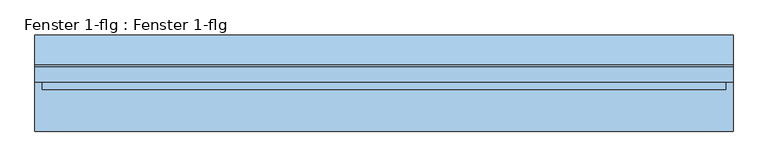
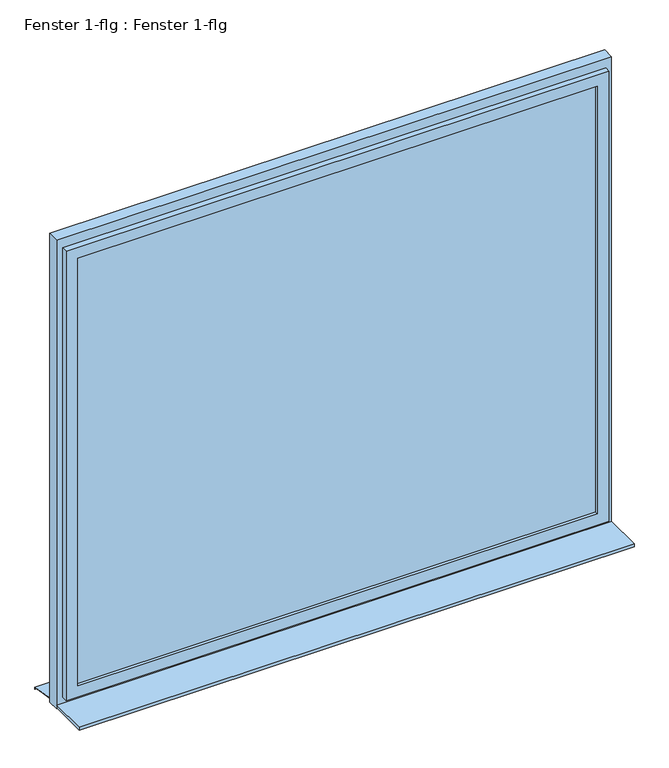
"""IFC4 building model written with IfcOpenShell, lengths in millimetres: window geometry, Fenster 1-flg : Fenster 1-flg."""

import ifcopenshell
import ifcopenshell.guid

model = None  # the IFC model being written
_history = None  # IfcOwnerHistory: only IFC2X3 demands one
_inside = {}  # id of a spatial element -> (the spatial element, [elements in it])
_under = {}  # id of a project, library or spatial element -> (it, [spatial elements below it])
_declared = {}  # id of a project -> (the project, [libraries it declares])
_typed = {}  # id of a type object -> (the type object, [elements of that type])
_made_of = {}  # id of a material, layer set ... -> (it, [elements and type objects made of it])


def new_model(schema):
    """Start an empty IFC model of exactly this schema.

    Asked for "IFC4X3", IfcOpenShell would pick the latest addendum, in which some entities
    have other attributes; the version numbers below select the first issue.
    IFC2X3 requires an IfcOwnerHistory on every rooted entity: one is made here for all.
    """
    global model, _history
    if schema == "IFC4X3":
        model = ifcopenshell.file(schema_version=(4, 3, 0, 0))
    else:
        model = ifcopenshell.file(schema=schema)
    _inside.clear()
    _under.clear()
    _declared.clear()
    _typed.clear()
    _made_of.clear()
    _history = None
    if model.schema == "IFC2X3":
        org = make("IfcOrganization", Name="unknown")
        user = make(
            "IfcPersonAndOrganization",
            ThePerson=make("IfcPerson", FamilyName="unknown"),
            TheOrganization=org,
        )
        app = make(
            "IfcApplication",
            ApplicationDeveloper=org,
            Version="unknown",
            ApplicationFullName="unknown",
            ApplicationIdentifier="unknown",
        )
        _history = make(
            "IfcOwnerHistory",
            OwningUser=user,
            OwningApplication=app,
            ChangeAction="ADDED",
            CreationDate=0,
        )
    return model


def make(cls, **values):
    """One entity of the class cls with the attributes given. An attribute that is None is left unset."""
    return model.create_entity(
        cls, **{name: value for name, value in values.items() if value is not None}
    )


def rooted(cls, **values):
    """An entity with a GlobalId (a new one), such as an element, a storey or a relation."""
    return make(cls, GlobalId=ifcopenshell.guid.new(), OwnerHistory=_history, **values)


def si_unit(unit_type, name, prefix=None):
    """IfcSIUnit, for example si_unit("LENGTHUNIT", "METRE", prefix="MILLI")."""
    return make("IfcSIUnit", UnitType=unit_type, Prefix=prefix, Name=name)


def assignment(units):
    """IfcUnitAssignment: the units of a project."""
    return None if units is None else make("IfcUnitAssignment", Units=units)


def point(xyz):
    """IfcCartesianPoint."""
    return None if xyz is None else make("IfcCartesianPoint", Coordinates=xyz)


def direction(xyz):
    """IfcDirection."""
    return None if xyz is None else make("IfcDirection", DirectionRatios=xyz)


def frame(location, z_axis=None, x_axis=None):
    """IfcAxis2Placement3D, a coordinate frame: its origin and axes. An axis left out is left unset."""
    return make(
        "IfcAxis2Placement3D",
        Location=point(location),
        Axis=direction(z_axis),
        RefDirection=direction(x_axis),
    )


def origin():
    """The frame at (0, 0, 0) with its axes left unset."""
    return frame((0.0, 0.0, 0.0))


def place(relative_to, where):
    """IfcLocalPlacement: puts the frame where relative to a parent placement (None: the world)."""
    return make(
        "IfcLocalPlacement", PlacementRelTo=relative_to, RelativePlacement=where
    )


def context(
    kind, dimensions, precision=None, world=None, true_north=None, identifier=None
):
    """IfcGeometricRepresentationContext, for example the 3D "Model" context."""
    return make(
        "IfcGeometricRepresentationContext",
        ContextIdentifier=identifier,
        ContextType=kind,
        CoordinateSpaceDimension=dimensions,
        Precision=precision,
        WorldCoordinateSystem=world,
        TrueNorth=true_north,
    )


def project(units=None, contexts=None):
    """IfcProject with its units and contexts."""
    return rooted(
        "IfcProject",
        Name="project",
        RepresentationContexts=contexts,
        UnitsInContext=assignment(units),
    )


def spatial(cls, under=None, at=None, **own):
    """A site, building, storey or space (cls), placed at a placement, below another one or the project."""
    s = rooted(cls, ObjectPlacement=at, **own)
    if under is not None:
        _under.setdefault(under.id(), (under, []))[1].append(s)
    return s


def polyline(points):
    """IfcPolyline through the points."""
    return make("IfcPolyline", Points=[point(p) for p in points])


def outline(outer, holes=None, kind="AREA"):
    """IfcArbitraryClosedProfileDef: a profile drawn as a closed curve; with holes, ...WithVoids."""
    if holes is None:
        return make("IfcArbitraryClosedProfileDef", ProfileType=kind, OuterCurve=outer)
    return make(
        "IfcArbitraryProfileDefWithVoids",
        ProfileType=kind,
        OuterCurve=outer,
        InnerCurves=holes,
    )


def extrude(swept, where, along, depth):
    """IfcExtrudedAreaSolid: the profile swept, set in the frame where, extruded along a direction by depth."""
    return make(
        "IfcExtrudedAreaSolid",
        SweptArea=swept,
        Position=where,
        ExtrudedDirection=direction(along),
        Depth=depth,
    )


def faces_of(points, faces, orient=None, outer=None):
    """IfcFace entities. A face is a list of loops; a loop is a list of indices into points, from 0.

    orient and outer hold one flag for each loop. By default every Orientation is true, the
    first loop of a face is its IfcFaceOuterBound and the others are IfcFaceBound.
    """
    made = []
    for i, loops in enumerate(faces):
        bounds = []
        for j, loop in enumerate(loops):
            is_outer = j == 0 if outer is None else outer[i][j]
            bounds.append(
                make(
                    "IfcFaceOuterBound" if is_outer else "IfcFaceBound",
                    Bound=make("IfcPolyLoop", Polygon=[points[k] for k in loop]),
                    Orientation=True if orient is None else orient[i][j],
                )
            )
        made.append(make("IfcFace", Bounds=bounds))
    return made


def faceted_brep(points, faces, orient=None, outer=None, voids=None):
    """IfcFacetedBrep: a solid bounded by flat faces; with voids (closed shells), ...WithVoids."""
    shared = [point(p) for p in points]
    hull = make("IfcClosedShell", CfsFaces=faces_of(shared, faces, orient, outer))
    if voids is None:
        return make("IfcFacetedBrep", Outer=hull)
    return make(
        "IfcFacetedBrepWithVoids",
        Outer=hull,
        Voids=[
            make(cls, CfsFaces=faces_of(shared, fs, o, b)) for cls, fs, o, b in voids
        ],
    )


def shape(context_of_items, identifier, shape_type, items):
    """IfcShapeRepresentation: the items that make up one representation, for example the "Body"."""
    return make(
        "IfcShapeRepresentation",
        ContextOfItems=context_of_items,
        RepresentationIdentifier=identifier,
        RepresentationType=shape_type,
        Items=items,
    )


def source(mapping_origin, context_of_items, identifier, shape_type, items):
    """IfcRepresentationMap: a shape defined once, which mapped items show again and again."""
    return make(
        "IfcRepresentationMap",
        MappingOrigin=mapping_origin,
        MappedRepresentation=shape(context_of_items, identifier, shape_type, items),
    )


def transform(
    local_origin,
    x_axis=None,
    y_axis=None,
    z_axis=None,
    scale=None,
    scale2=None,
    scale3=None,
    uniform=True,
):
    """IfcCartesianTransformationOperator3D, or its non-uniform kind. x_axis, y_axis, z_axis: its Axis1, 2, 3."""
    if uniform:
        return make(
            "IfcCartesianTransformationOperator3D",
            Axis1=direction(x_axis),
            Axis2=direction(y_axis),
            LocalOrigin=point(local_origin),
            Scale=scale,
            Axis3=direction(z_axis),
        )
    return make(
        "IfcCartesianTransformationOperator3DnonUniform",
        Axis1=direction(x_axis),
        Axis2=direction(y_axis),
        LocalOrigin=point(local_origin),
        Scale=scale,
        Axis3=direction(z_axis),
        Scale2=scale2,
        Scale3=scale3,
    )


def mapped(mapping_source, mapping_target):
    """IfcMappedItem: shows the shape of a source again, moved by a transform."""
    return make(
        "IfcMappedItem", MappingSource=mapping_source, MappingTarget=mapping_target
    )


def made_of(thing, what):
    """Note that an element or type object is made of a material, layer set ...; save() writes the relation."""
    if what is not None:
        _made_of.setdefault(what.id(), (what, []))[1].append(thing)
    return thing


def element(
    cls,
    number,
    at=None,
    inside=None,
    cuts=None,
    type_object=None,
    material=None,
    context=None,
    identifier="Body",
    shape_type=None,
    held_by="IfcProductDefinitionShape",
    body=None,
    shapes=None,
    **own,
):
    """One element of the class cls, such as IfcWall. Its Tag is "e" and its number.

    at: its placement. inside: the storey or other place that contains it. cuts: it is an
    opening in that element (IfcRelVoidsElement). A single representation is given by context,
    identifier, shape_type and body (its items); several are given by shapes. held_by: the class
    of the entity that holds the representations. save() writes the other relations.
    """
    e = rooted(cls, Tag="e%d" % number, ObjectPlacement=at, **own)
    if body is not None:
        shapes = [shape(context, identifier, shape_type, body)]
    if shapes is not None:
        e.Representation = make(held_by, Representations=shapes)
    if inside is not None:
        _inside.setdefault(inside.id(), (inside, []))[1].append(e)
    if cuts is not None:
        rooted(
            "IfcRelVoidsElement", RelatingBuildingElement=cuts, RelatedOpeningElement=e
        )
    if type_object is not None:
        _typed.setdefault(type_object.id(), (type_object, []))[1].append(e)
    return made_of(e, material)


def aggregate(whole, parts):
    """IfcRelAggregates: a whole, such as a stair, and the parts it consists of."""
    return rooted("IfcRelAggregates", RelatingObject=whole, RelatedObjects=parts)


def save(model, path):
    """Write the relations noted so far, then the file.

    IfcRelAggregates (storeys below a building ...), IfcRelContainedInSpatialStructure (elements
    in a storey), IfcRelDefinesByType, IfcRelAssociatesMaterial and IfcRelDeclares: one each for
    every whole, place, type object, material and project.
    """
    for whole, parts in _under.values():
        aggregate(whole, parts)
    for where, things in _inside.values():
        rooted(
            "IfcRelContainedInSpatialStructure",
            RelatedElements=things,
            RelatingStructure=where,
        )
    for kind, things in _typed.values():
        rooted("IfcRelDefinesByType", RelatedObjects=things, RelatingType=kind)
    for what, things in _made_of.values():
        rooted("IfcRelAssociatesMaterial", RelatedObjects=things, RelatingMaterial=what)
    for by, libraries in _declared.values():
        rooted("IfcRelDeclares", RelatingContext=by, RelatedDefinitions=libraries)
    model.write(path)


def fenster_1_flg_fenster_1_flg_fbf7811f(model_context):
    return source(origin(), model_context, "Body", "SolidModel", [
        extrude(outline(polyline([(3500.0, 1400.0), (3500.0, -1400.0), (1000.0, -1400.0), (1000.0, 1400.0), (3500.0, 1400.0)]), holes=[polyline([(3420.0, 1340.0), (1080.0, 1340.0), (1080.0, -1340.0), (3420.0, -1340.0), (3420.0, 1340.0)])]), frame((0.0, 3.5, 0.0), z_axis=(0.0, 1.0, 0.0), x_axis=(0.0, 0.0, 1.0)), (0.0, 0.0, 1.0), 60.0),
        faceted_brep([(1370.0, 3.5, 3450.0), (1370.0, -26.5, 3450.0), (1370.0, -26.5, 1050.0), (1370.0, 3.5, 1050.0), (-1370.0, -26.5, 3450.0), (-1370.0, -26.5, 1050.0), (1310.0, -26.5, 1110.0), (-1310.0, -26.5, 1110.0), (-1310.0, -26.5, 3390.0), (1310.0, -26.5, 3390.0), (-1370.0, 3.5, 1050.0), (-1370.0, 3.5, 3450.0), (1340.0, 3.5, 3420.0), (-1340.0, 3.5, 3420.0), (-1340.0, 3.5, 1080.0), (1340.0, 3.5, 1080.0), (1340.0, 33.5, 3420.0), (1340.0, 33.5, 1080.0), (-1340.0, 33.5, 1080.0), (-1340.0, 33.5, 3420.0), (1310.0, 33.5, 3390.0), (-1310.0, 33.5, 3390.0), (-1310.0, 33.5, 1110.0), (1310.0, 33.5, 1110.0)], [[[0, 1, 2, 3]], [[1, 4, 5, 2], [6, 7, 8, 9]], [[3, 2, 5, 10]], [[3, 10, 11, 0], [12, 13, 14, 15]], [[16, 12, 15, 17]], [[17, 15, 14, 18]], [[17, 18, 19, 16], [20, 21, 22, 23]], [[9, 20, 23, 6]], [[6, 23, 22, 7]], [[10, 5, 4, 11]], [[18, 14, 13, 19]], [[7, 22, 21, 8]], [[11, 4, 1, 0]], [[19, 13, 12, 16]], [[8, 21, 20, 9]]]),
        extrude(outline(polyline([(-1400.0, -193.5), (-1400.0, 3.5), (1400.0, 3.5), (1400.0, -193.5), (-1400.0, -193.5)])), frame((0.0, 0.0, 1005.0), z_axis=(0.0, 0.0, 1.0), x_axis=(1.0, 0.0, 0.0)), (0.0, 0.0, 1.0), 15.0),
        extrude(outline(polyline([(73.5221543, 1020.0), (193.5, 1000.0), (193.5, 990.0), (191.5, 990.0), (191.5, 998.3604634), (73.3240723, 1018.0), (63.5, 1018.0), (63.5, 1020.0), (73.5221543, 1020.0)])), frame((-1400.0, 0.0, 0.0), z_axis=(1.0, 0.0, 0.0), x_axis=(0.0, 1.0, 0.0)), (0.0, 0.0, 1.0), 2800.0),
        extrude(outline(polyline([(1310.0, -11.5), (-1310.0, -11.5), (-1310.0, 18.5), (1310.0, 18.5), (1310.0, -11.5)])), frame((0.0, 0.0, 1110.0), z_axis=(0.0, 0.0, 1.0), x_axis=(1.0, 0.0, 0.0)), (0.0, 0.0, 1.0), 2280.0),
    ])


if __name__ == "__main__":
    model = new_model("IFC4")
    model_context = context("Model", 3, world=origin())
    ifc_project = project(units=[si_unit("LENGTHUNIT", "METRE", prefix="MILLI")], contexts=[model_context])
    site = spatial("IfcSite", under=ifc_project)
    building = spatial("IfcBuilding", under=site)
    placement = place(None, origin())
    fenster_1_flg_fenster_1_flg_shape = fenster_1_flg_fenster_1_flg_fbf7811f(model_context)
    element("IfcWindow", 1, ObjectType="Fenster 1-flg : Fenster 1-flg", at=placement, inside=building, context=model_context, shape_type="MappedRepresentation", body=[
        mapped(fenster_1_flg_fenster_1_flg_shape, transform((0.0, 0.0, 0.0), x_axis=(1.0, 0.0, 0.0), y_axis=(0.0, 1.0, 0.0), z_axis=(0.0, 0.0, 1.0))),
    ])
    save(model, "model.ifc")

# Revit data of these elements
# Project information
#   Project Issue Date = "Ausgabedatum"
#   Project Status = "Projektstatus"
#   Client Name = "Besitzer"
#   Project Address = "Geben Sie die Adresse hier ein"
#   Project Name = "Projektname"
#   Project Number = "Projektnummer"
#   magiDataSet = "C:\\ProgramData\\MagiCAD-RS\\2014_r2014\\Datasets\\Common\\Common-MCREV-2014_11a_r2014.mrv"
#   magiVersionCreated = "2014.11"
#   magiVersionSaved = "2014.11"
#   magiParamsCreated = "2014.11"
# Type "Fenster 1-flg : Fenster 1-flg"
#   Type Mark = "45"
#   Operation = "SinglePanel"
#   Construction Type Id = "RGDPK6R"
#   Keynote = "16.05.01"
#   Analytic Construction = "Low-E double glazing (1/4 in + 1/4 in)"
#   Visual Light Transmittance = 0.76
#   Thermal Resistance (R) = 0.179801 (m²·K)/W
#   Solar Heat Gain Coefficient = 0.65
#   Rough Width = 2800 mm
#   Rough Height = 2500 mm
#   Heat Transfer Coefficient (U) = 2.1030 W/(m²·K)
#   Rahmentiefe = 60 mm
#   Rahmenhöhe unten = 80 mm
#   Rahmenhöhe oben = 80 mm
#   Rahmenbreite = 60 mm
#   Height = 2500 mm
#   Flügeltiefe = 60 mm
#   Flügelbreite = 60 mm
#   Einbautiefe (von außen) [instance default] = 100 mm
#   Width = 2800 mm
#   Klappflügel [instance default] = no
#   Kippflügel [instance default] = yes
#   Öffnungsrichtung in Draufsicht anzeigen [instance default] = no
#   Drehflügel [instance default] = yes
#   Rahmen [instance default] = none
#   Glas [instance default] = none
#   Lüftungsöffnung [instance default] = none
#   Fensterbank innen [instance default] = none
#   Fensterbank außen [instance default] = none
#   Wall Closure = (empty or 0)
# Element 1 (IfcWindow, "Fenster 1-flg : Fenster 1-flg")
#   Materials on its faces: "Fenster - Kunststoff weiß", "Farbe Grau", "Glas", "Farbe Weiss", "Fenster - Holz"
# Materials
#   "Fenster - Kunststoff weiß": class "Kunststoff", colour RGB 249 249 249, transparency 0
#   "Farbe Grau": class "Generic", colour RGB 85 85 85, transparency 0, Cost = 0
#   "Glas": class "Glas", colour RGB 0 128 192, transparency 0.75, Description = "Kalknatronglas", Cost = 0
#   "Farbe Weiss": class "Generic", colour RGB 255 255 255, transparency 0, Cost = 0
#   "Fenster - Holz": class "Holz", colour RGB 216 135 75, transparency 0
